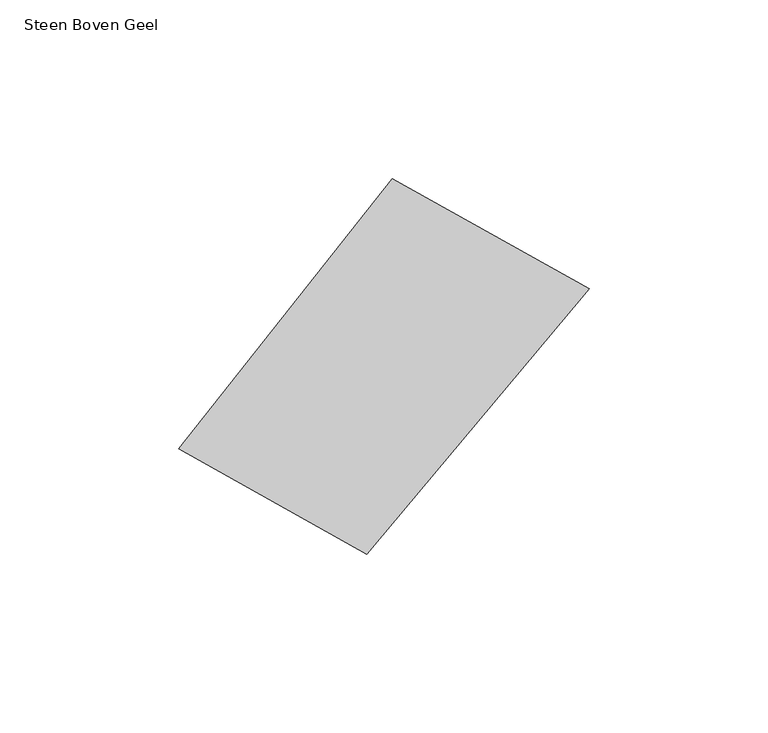
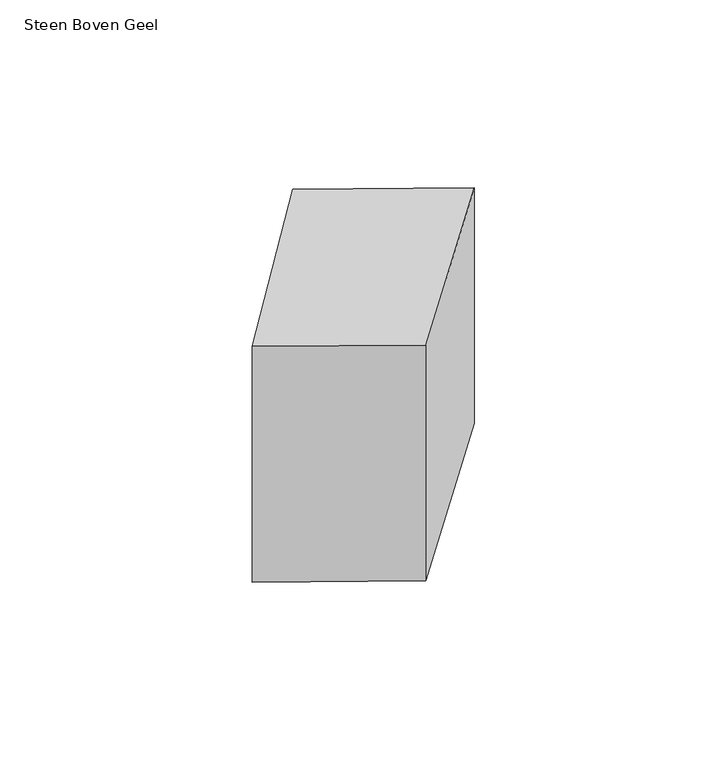
"""IFC4 building model written with IfcOpenShell, lengths in millimetres: proxy geometry, 00_GMA_steen_versie_4 : Steen Boven Geel."""

from ifc_helpers import new_model, si_unit, origin, origin_with_axes, place, context, project, spatial, polyline, outline, extrude, source, transform, mapped, element, save


def steen_boven_geel_a1c3697e(model_context):
    return source(origin(), model_context, "Body", "SweptSolid", [
        extrude(outline(polyline([(164.6581315, 73.7201968), (102.4599039, -0.4361196), (49.8539995, 29.024444), (109.6129641, 104.5216218), (164.6581315, 73.7201968)])), origin_with_axes(), (0.0, 0.0, 1.0), 100.0),
    ])


if __name__ == "__main__":
    model = new_model("IFC4")
    model_context = context("Model", 3, world=origin())
    ifc_project = project(units=[si_unit("LENGTHUNIT", "METRE", prefix="MILLI")], contexts=[model_context])
    site = spatial("IfcSite", under=ifc_project)
    building = spatial("IfcBuilding", under=site)
    placement = place(None, origin())
    steen_boven_geel_shape = steen_boven_geel_a1c3697e(model_context)
    element("IfcBuildingElementProxy", 1, Name="00_GMA_steen_versie_4 : Steen Boven Geel", ObjectType="00_GMA_steen_versie_4 : Steen Boven Geel", at=placement, inside=building, context=model_context, shape_type="MappedRepresentation", body=[
        mapped(steen_boven_geel_shape, transform((0.0, 0.0, 0.0), x_axis=(1.0, 0.0, 0.0), y_axis=(0.0, 1.0, 0.0), z_axis=(0.0, 0.0, 1.0))),
    ])
    save(model, "model.ifc")

# Revit data of these elements
# Type "00_GMA_steen_versie_4 : Steen Boven Geel"
#   StootVoegHalfBoven [instance default] = 5 mm
#   StootVoegHalf [instance default] = 5 mm
#   StootVoegBreedteOnder = 10 mm
#   StootVoegBreedteBoven = 10 mm
#   Steendikte = 100 mm
#   LintVoegOnderHalf = 5 mm
#   LintVoegOnder = 10 mm
#   LintVoegBovenHalf = 0 mm
#   LintVoegBoven = 0 mm
#   materiaal = 21_steen_geel
#   MateriaalVoeg = none
#   Default Elevation = 0
# Element 1 (IfcBuildingElementProxy, "00_GMA_steen_versie_4 : Steen Boven Geel")
#   Materials on its faces: "21_steen_geel"
# Materials
#   "21_steen_geel": class "Unassigned", colour RGB 202 202 0, transparency 0, Cost = 0
